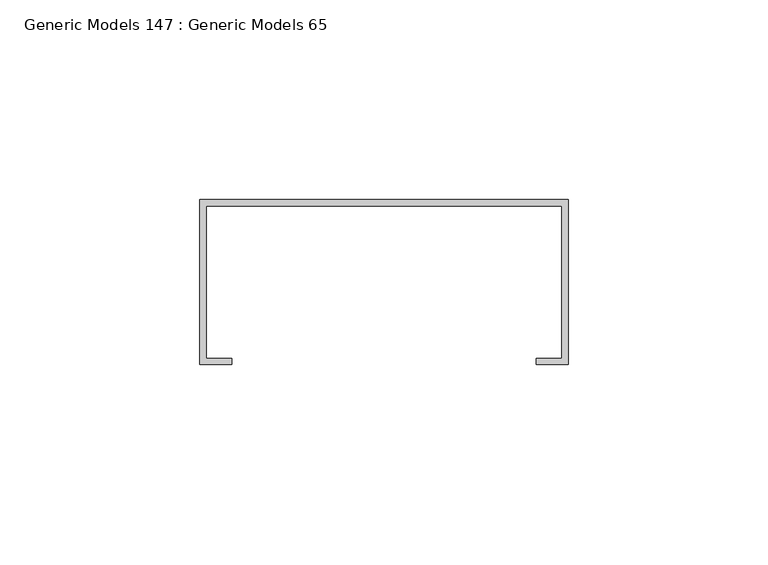
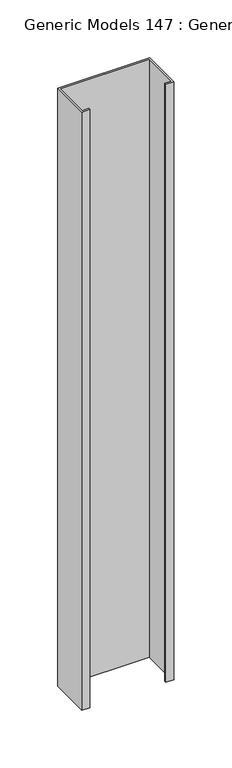
"""IFC4 building model written with IfcOpenShell, lengths in millimetres: proxy geometry, Generic Models 147 : Generic Models 65."""

import ifcopenshell
import ifcopenshell.guid

model = None  # the IFC model being written
_history = None  # IfcOwnerHistory: only IFC2X3 demands one
_inside = {}  # id of a spatial element -> (the spatial element, [elements in it])
_under = {}  # id of a project, library or spatial element -> (it, [spatial elements below it])
_declared = {}  # id of a project -> (the project, [libraries it declares])
_typed = {}  # id of a type object -> (the type object, [elements of that type])
_made_of = {}  # id of a material, layer set ... -> (it, [elements and type objects made of it])


def new_model(schema):
    """Start an empty IFC model of exactly this schema.

    Asked for "IFC4X3", IfcOpenShell would pick the latest addendum, in which some entities
    have other attributes; the version numbers below select the first issue.
    IFC2X3 requires an IfcOwnerHistory on every rooted entity: one is made here for all.
    """
    global model, _history
    if schema == "IFC4X3":
        model = ifcopenshell.file(schema_version=(4, 3, 0, 0))
    else:
        model = ifcopenshell.file(schema=schema)
    _inside.clear()
    _under.clear()
    _declared.clear()
    _typed.clear()
    _made_of.clear()
    _history = None
    if model.schema == "IFC2X3":
        org = make("IfcOrganization", Name="unknown")
        user = make(
            "IfcPersonAndOrganization",
            ThePerson=make("IfcPerson", FamilyName="unknown"),
            TheOrganization=org,
        )
        app = make(
            "IfcApplication",
            ApplicationDeveloper=org,
            Version="unknown",
            ApplicationFullName="unknown",
            ApplicationIdentifier="unknown",
        )
        _history = make(
            "IfcOwnerHistory",
            OwningUser=user,
            OwningApplication=app,
            ChangeAction="ADDED",
            CreationDate=0,
        )
    return model


def make(cls, **values):
    """One entity of the class cls with the attributes given. An attribute that is None is left unset."""
    return model.create_entity(
        cls, **{name: value for name, value in values.items() if value is not None}
    )


def rooted(cls, **values):
    """An entity with a GlobalId (a new one), such as an element, a storey or a relation."""
    return make(cls, GlobalId=ifcopenshell.guid.new(), OwnerHistory=_history, **values)


def si_unit(unit_type, name, prefix=None):
    """IfcSIUnit, for example si_unit("LENGTHUNIT", "METRE", prefix="MILLI")."""
    return make("IfcSIUnit", UnitType=unit_type, Prefix=prefix, Name=name)


def assignment(units):
    """IfcUnitAssignment: the units of a project."""
    return None if units is None else make("IfcUnitAssignment", Units=units)


def point(xyz):
    """IfcCartesianPoint."""
    return None if xyz is None else make("IfcCartesianPoint", Coordinates=xyz)


def direction(xyz):
    """IfcDirection."""
    return None if xyz is None else make("IfcDirection", DirectionRatios=xyz)


def frame(location, z_axis=None, x_axis=None):
    """IfcAxis2Placement3D, a coordinate frame: its origin and axes. An axis left out is left unset."""
    return make(
        "IfcAxis2Placement3D",
        Location=point(location),
        Axis=direction(z_axis),
        RefDirection=direction(x_axis),
    )


def origin():
    """The frame at (0, 0, 0) with its axes left unset."""
    return frame((0.0, 0.0, 0.0))


def place(relative_to, where):
    """IfcLocalPlacement: puts the frame where relative to a parent placement (None: the world)."""
    return make(
        "IfcLocalPlacement", PlacementRelTo=relative_to, RelativePlacement=where
    )


def context(
    kind, dimensions, precision=None, world=None, true_north=None, identifier=None
):
    """IfcGeometricRepresentationContext, for example the 3D "Model" context."""
    return make(
        "IfcGeometricRepresentationContext",
        ContextIdentifier=identifier,
        ContextType=kind,
        CoordinateSpaceDimension=dimensions,
        Precision=precision,
        WorldCoordinateSystem=world,
        TrueNorth=true_north,
    )


def project(units=None, contexts=None):
    """IfcProject with its units and contexts."""
    return rooted(
        "IfcProject",
        Name="project",
        RepresentationContexts=contexts,
        UnitsInContext=assignment(units),
    )


def spatial(cls, under=None, at=None, **own):
    """A site, building, storey or space (cls), placed at a placement, below another one or the project."""
    s = rooted(cls, ObjectPlacement=at, **own)
    if under is not None:
        _under.setdefault(under.id(), (under, []))[1].append(s)
    return s


def polyline(points):
    """IfcPolyline through the points."""
    return make("IfcPolyline", Points=[point(p) for p in points])


def outline(outer, holes=None, kind="AREA"):
    """IfcArbitraryClosedProfileDef: a profile drawn as a closed curve; with holes, ...WithVoids."""
    if holes is None:
        return make("IfcArbitraryClosedProfileDef", ProfileType=kind, OuterCurve=outer)
    return make(
        "IfcArbitraryProfileDefWithVoids",
        ProfileType=kind,
        OuterCurve=outer,
        InnerCurves=holes,
    )


def extrude(swept, where, along, depth):
    """IfcExtrudedAreaSolid: the profile swept, set in the frame where, extruded along a direction by depth."""
    return make(
        "IfcExtrudedAreaSolid",
        SweptArea=swept,
        Position=where,
        ExtrudedDirection=direction(along),
        Depth=depth,
    )


def shape(context_of_items, identifier, shape_type, items):
    """IfcShapeRepresentation: the items that make up one representation, for example the "Body"."""
    return make(
        "IfcShapeRepresentation",
        ContextOfItems=context_of_items,
        RepresentationIdentifier=identifier,
        RepresentationType=shape_type,
        Items=items,
    )


def source(mapping_origin, context_of_items, identifier, shape_type, items):
    """IfcRepresentationMap: a shape defined once, which mapped items show again and again."""
    return make(
        "IfcRepresentationMap",
        MappingOrigin=mapping_origin,
        MappedRepresentation=shape(context_of_items, identifier, shape_type, items),
    )


def transform(
    local_origin,
    x_axis=None,
    y_axis=None,
    z_axis=None,
    scale=None,
    scale2=None,
    scale3=None,
    uniform=True,
):
    """IfcCartesianTransformationOperator3D, or its non-uniform kind. x_axis, y_axis, z_axis: its Axis1, 2, 3."""
    if uniform:
        return make(
            "IfcCartesianTransformationOperator3D",
            Axis1=direction(x_axis),
            Axis2=direction(y_axis),
            LocalOrigin=point(local_origin),
            Scale=scale,
            Axis3=direction(z_axis),
        )
    return make(
        "IfcCartesianTransformationOperator3DnonUniform",
        Axis1=direction(x_axis),
        Axis2=direction(y_axis),
        LocalOrigin=point(local_origin),
        Scale=scale,
        Axis3=direction(z_axis),
        Scale2=scale2,
        Scale3=scale3,
    )


def mapped(mapping_source, mapping_target):
    """IfcMappedItem: shows the shape of a source again, moved by a transform."""
    return make(
        "IfcMappedItem", MappingSource=mapping_source, MappingTarget=mapping_target
    )


def made_of(thing, what):
    """Note that an element or type object is made of a material, layer set ...; save() writes the relation."""
    if what is not None:
        _made_of.setdefault(what.id(), (what, []))[1].append(thing)
    return thing


def element(
    cls,
    number,
    at=None,
    inside=None,
    cuts=None,
    type_object=None,
    material=None,
    context=None,
    identifier="Body",
    shape_type=None,
    held_by="IfcProductDefinitionShape",
    body=None,
    shapes=None,
    **own,
):
    """One element of the class cls, such as IfcWall. Its Tag is "e" and its number.

    at: its placement. inside: the storey or other place that contains it. cuts: it is an
    opening in that element (IfcRelVoidsElement). A single representation is given by context,
    identifier, shape_type and body (its items); several are given by shapes. held_by: the class
    of the entity that holds the representations. save() writes the other relations.
    """
    e = rooted(cls, Tag="e%d" % number, ObjectPlacement=at, **own)
    if body is not None:
        shapes = [shape(context, identifier, shape_type, body)]
    if shapes is not None:
        e.Representation = make(held_by, Representations=shapes)
    if inside is not None:
        _inside.setdefault(inside.id(), (inside, []))[1].append(e)
    if cuts is not None:
        rooted(
            "IfcRelVoidsElement", RelatingBuildingElement=cuts, RelatedOpeningElement=e
        )
    if type_object is not None:
        _typed.setdefault(type_object.id(), (type_object, []))[1].append(e)
    return made_of(e, material)


def aggregate(whole, parts):
    """IfcRelAggregates: a whole, such as a stair, and the parts it consists of."""
    return rooted("IfcRelAggregates", RelatingObject=whole, RelatedObjects=parts)


def save(model, path):
    """Write the relations noted so far, then the file.

    IfcRelAggregates (storeys below a building ...), IfcRelContainedInSpatialStructure (elements
    in a storey), IfcRelDefinesByType, IfcRelAssociatesMaterial and IfcRelDeclares: one each for
    every whole, place, type object, material and project.
    """
    for whole, parts in _under.values():
        aggregate(whole, parts)
    for where, things in _inside.values():
        rooted(
            "IfcRelContainedInSpatialStructure",
            RelatedElements=things,
            RelatingStructure=where,
        )
    for kind, things in _typed.values():
        rooted("IfcRelDefinesByType", RelatedObjects=things, RelatingType=kind)
    for what, things in _made_of.values():
        rooted("IfcRelAssociatesMaterial", RelatedObjects=things, RelatingMaterial=what)
    for by, libraries in _declared.values():
        rooted("IfcRelDeclares", RelatingContext=by, RelatedDefinitions=libraries)
    model.write(path)


def generic_models_147_generic_models_65_fc30ab23(model_context):
    return source(origin(), model_context, "Body", "SweptSolid", [
        extrude(outline(polyline([(48062.9985531, 630.2375), (48155.0735531, 630.2375), (48155.0735531, 588.9625), (48147.1360531, 588.9625), (48147.1360531, 590.55), (48153.4860531, 590.55), (48153.4860531, 628.65), (48064.5860531, 628.65), (48064.5860531, 590.55), (48070.9360531, 590.55), (48070.9360531, 588.9625), (48062.9985531, 588.9625), (48062.9985531, 630.2375)])), frame((0.0, 0.0, 1598.2598705), z_axis=(0.0, 0.0, 1.0), x_axis=(1.0, 0.0, 0.0)), (0.0, 0.0, 1.0), 631.6265625),
    ])


if __name__ == "__main__":
    model = new_model("IFC4")
    model_context = context("Model", 3, world=origin())
    ifc_project = project(units=[si_unit("LENGTHUNIT", "METRE", prefix="MILLI")], contexts=[model_context])
    site = spatial("IfcSite", under=ifc_project)
    building = spatial("IfcBuilding", under=site)
    placement = place(None, origin())
    generic_models_147_generic_models_65_shape = generic_models_147_generic_models_65_fc30ab23(model_context)
    element("IfcBuildingElementProxy", 1, Name="Generic Models 147 : Generic Models 65", ObjectType="Generic Models 147 : Generic Models 65", at=placement, inside=building, context=model_context, shape_type="MappedRepresentation", body=[
        mapped(generic_models_147_generic_models_65_shape, transform((0.0, 0.0, 0.0), x_axis=(1.0, 0.0, 0.0), y_axis=(0.0, 1.0, 0.0), z_axis=(0.0, 0.0, 1.0))),
    ])
    save(model, "model.ifc")

# Revit data of these elements
# Element 1 (IfcBuildingElementProxy, "Generic Models 147 : Generic Models 65")
#   Materials on its faces: "METAL STUD (16\" O.C.)"
# Materials
#   "METAL STUD (16\" O.C.)": class "Unassigned", colour RGB 210 209 208, transparency 0, Keynote = "M05121300.02", Cost = 0
